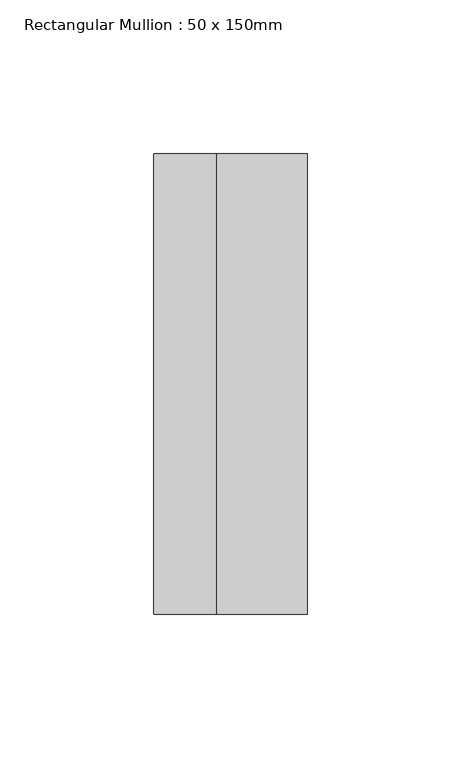
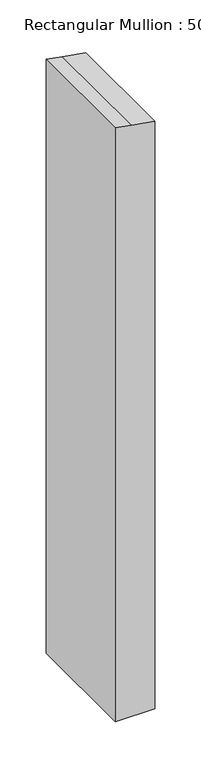
"""IFC4 building model written with IfcOpenShell, lengths in millimetres: member geometry, Rectangular Mullion : 50 x 150mm."""

import ifcopenshell
import ifcopenshell.guid

model = None  # the IFC model being written
_history = None  # IfcOwnerHistory: only IFC2X3 demands one
_inside = {}  # id of a spatial element -> (the spatial element, [elements in it])
_under = {}  # id of a project, library or spatial element -> (it, [spatial elements below it])
_declared = {}  # id of a project -> (the project, [libraries it declares])
_typed = {}  # id of a type object -> (the type object, [elements of that type])
_made_of = {}  # id of a material, layer set ... -> (it, [elements and type objects made of it])


def new_model(schema):
    """Start an empty IFC model of exactly this schema.

    Asked for "IFC4X3", IfcOpenShell would pick the latest addendum, in which some entities
    have other attributes; the version numbers below select the first issue.
    IFC2X3 requires an IfcOwnerHistory on every rooted entity: one is made here for all.
    """
    global model, _history
    if schema == "IFC4X3":
        model = ifcopenshell.file(schema_version=(4, 3, 0, 0))
    else:
        model = ifcopenshell.file(schema=schema)
    _inside.clear()
    _under.clear()
    _declared.clear()
    _typed.clear()
    _made_of.clear()
    _history = None
    if model.schema == "IFC2X3":
        org = make("IfcOrganization", Name="unknown")
        user = make(
            "IfcPersonAndOrganization",
            ThePerson=make("IfcPerson", FamilyName="unknown"),
            TheOrganization=org,
        )
        app = make(
            "IfcApplication",
            ApplicationDeveloper=org,
            Version="unknown",
            ApplicationFullName="unknown",
            ApplicationIdentifier="unknown",
        )
        _history = make(
            "IfcOwnerHistory",
            OwningUser=user,
            OwningApplication=app,
            ChangeAction="ADDED",
            CreationDate=0,
        )
    return model


def make(cls, **values):
    """One entity of the class cls with the attributes given. An attribute that is None is left unset."""
    return model.create_entity(
        cls, **{name: value for name, value in values.items() if value is not None}
    )


def rooted(cls, **values):
    """An entity with a GlobalId (a new one), such as an element, a storey or a relation."""
    return make(cls, GlobalId=ifcopenshell.guid.new(), OwnerHistory=_history, **values)


def si_unit(unit_type, name, prefix=None):
    """IfcSIUnit, for example si_unit("LENGTHUNIT", "METRE", prefix="MILLI")."""
    return make("IfcSIUnit", UnitType=unit_type, Prefix=prefix, Name=name)


def assignment(units):
    """IfcUnitAssignment: the units of a project."""
    return None if units is None else make("IfcUnitAssignment", Units=units)


def point(xyz):
    """IfcCartesianPoint."""
    return None if xyz is None else make("IfcCartesianPoint", Coordinates=xyz)


def direction(xyz):
    """IfcDirection."""
    return None if xyz is None else make("IfcDirection", DirectionRatios=xyz)


def frame(location, z_axis=None, x_axis=None):
    """IfcAxis2Placement3D, a coordinate frame: its origin and axes. An axis left out is left unset."""
    return make(
        "IfcAxis2Placement3D",
        Location=point(location),
        Axis=direction(z_axis),
        RefDirection=direction(x_axis),
    )


def origin():
    """The frame at (0, 0, 0) with its axes left unset."""
    return frame((0.0, 0.0, 0.0))


def place(relative_to, where):
    """IfcLocalPlacement: puts the frame where relative to a parent placement (None: the world)."""
    return make(
        "IfcLocalPlacement", PlacementRelTo=relative_to, RelativePlacement=where
    )


def context(
    kind, dimensions, precision=None, world=None, true_north=None, identifier=None
):
    """IfcGeometricRepresentationContext, for example the 3D "Model" context."""
    return make(
        "IfcGeometricRepresentationContext",
        ContextIdentifier=identifier,
        ContextType=kind,
        CoordinateSpaceDimension=dimensions,
        Precision=precision,
        WorldCoordinateSystem=world,
        TrueNorth=true_north,
    )


def project(units=None, contexts=None):
    """IfcProject with its units and contexts."""
    return rooted(
        "IfcProject",
        Name="project",
        RepresentationContexts=contexts,
        UnitsInContext=assignment(units),
    )


def spatial(cls, under=None, at=None, **own):
    """A site, building, storey or space (cls), placed at a placement, below another one or the project."""
    s = rooted(cls, ObjectPlacement=at, **own)
    if under is not None:
        _under.setdefault(under.id(), (under, []))[1].append(s)
    return s


def polyline(points):
    """IfcPolyline through the points."""
    return make("IfcPolyline", Points=[point(p) for p in points])


def outline(outer, holes=None, kind="AREA"):
    """IfcArbitraryClosedProfileDef: a profile drawn as a closed curve; with holes, ...WithVoids."""
    if holes is None:
        return make("IfcArbitraryClosedProfileDef", ProfileType=kind, OuterCurve=outer)
    return make(
        "IfcArbitraryProfileDefWithVoids",
        ProfileType=kind,
        OuterCurve=outer,
        InnerCurves=holes,
    )


def extrude(swept, where, along, depth):
    """IfcExtrudedAreaSolid: the profile swept, set in the frame where, extruded along a direction by depth."""
    return make(
        "IfcExtrudedAreaSolid",
        SweptArea=swept,
        Position=where,
        ExtrudedDirection=direction(along),
        Depth=depth,
    )


def shape(context_of_items, identifier, shape_type, items):
    """IfcShapeRepresentation: the items that make up one representation, for example the "Body"."""
    return make(
        "IfcShapeRepresentation",
        ContextOfItems=context_of_items,
        RepresentationIdentifier=identifier,
        RepresentationType=shape_type,
        Items=items,
    )


def source(mapping_origin, context_of_items, identifier, shape_type, items):
    """IfcRepresentationMap: a shape defined once, which mapped items show again and again."""
    return make(
        "IfcRepresentationMap",
        MappingOrigin=mapping_origin,
        MappedRepresentation=shape(context_of_items, identifier, shape_type, items),
    )


def transform(
    local_origin,
    x_axis=None,
    y_axis=None,
    z_axis=None,
    scale=None,
    scale2=None,
    scale3=None,
    uniform=True,
):
    """IfcCartesianTransformationOperator3D, or its non-uniform kind. x_axis, y_axis, z_axis: its Axis1, 2, 3."""
    if uniform:
        return make(
            "IfcCartesianTransformationOperator3D",
            Axis1=direction(x_axis),
            Axis2=direction(y_axis),
            LocalOrigin=point(local_origin),
            Scale=scale,
            Axis3=direction(z_axis),
        )
    return make(
        "IfcCartesianTransformationOperator3DnonUniform",
        Axis1=direction(x_axis),
        Axis2=direction(y_axis),
        LocalOrigin=point(local_origin),
        Scale=scale,
        Axis3=direction(z_axis),
        Scale2=scale2,
        Scale3=scale3,
    )


def mapped(mapping_source, mapping_target):
    """IfcMappedItem: shows the shape of a source again, moved by a transform."""
    return make(
        "IfcMappedItem", MappingSource=mapping_source, MappingTarget=mapping_target
    )


def made_of(thing, what):
    """Note that an element or type object is made of a material, layer set ...; save() writes the relation."""
    if what is not None:
        _made_of.setdefault(what.id(), (what, []))[1].append(thing)
    return thing


def element(
    cls,
    number,
    at=None,
    inside=None,
    cuts=None,
    type_object=None,
    material=None,
    context=None,
    identifier="Body",
    shape_type=None,
    held_by="IfcProductDefinitionShape",
    body=None,
    shapes=None,
    **own,
):
    """One element of the class cls, such as IfcWall. Its Tag is "e" and its number.

    at: its placement. inside: the storey or other place that contains it. cuts: it is an
    opening in that element (IfcRelVoidsElement). A single representation is given by context,
    identifier, shape_type and body (its items); several are given by shapes. held_by: the class
    of the entity that holds the representations. save() writes the other relations.
    """
    e = rooted(cls, Tag="e%d" % number, ObjectPlacement=at, **own)
    if body is not None:
        shapes = [shape(context, identifier, shape_type, body)]
    if shapes is not None:
        e.Representation = make(held_by, Representations=shapes)
    if inside is not None:
        _inside.setdefault(inside.id(), (inside, []))[1].append(e)
    if cuts is not None:
        rooted(
            "IfcRelVoidsElement", RelatingBuildingElement=cuts, RelatedOpeningElement=e
        )
    if type_object is not None:
        _typed.setdefault(type_object.id(), (type_object, []))[1].append(e)
    return made_of(e, material)


def aggregate(whole, parts):
    """IfcRelAggregates: a whole, such as a stair, and the parts it consists of."""
    return rooted("IfcRelAggregates", RelatingObject=whole, RelatedObjects=parts)


def save(model, path):
    """Write the relations noted so far, then the file.

    IfcRelAggregates (storeys below a building ...), IfcRelContainedInSpatialStructure (elements
    in a storey), IfcRelDefinesByType, IfcRelAssociatesMaterial and IfcRelDeclares: one each for
    every whole, place, type object, material and project.
    """
    for whole, parts in _under.values():
        aggregate(whole, parts)
    for where, things in _inside.values():
        rooted(
            "IfcRelContainedInSpatialStructure",
            RelatedElements=things,
            RelatingStructure=where,
        )
    for kind, things in _typed.values():
        rooted("IfcRelDefinesByType", RelatedObjects=things, RelatingType=kind)
    for what, things in _made_of.values():
        rooted("IfcRelAssociatesMaterial", RelatedObjects=things, RelatingMaterial=what)
    for by, libraries in _declared.values():
        rooted("IfcRelDeclares", RelatingContext=by, RelatedDefinitions=libraries)
    model.write(path)


def rectangular_mullion_50_x_150mm_6a3808df(model_context):
    return source(origin(), model_context, "Body", "SweptSolid", [
        extrude(outline(polyline([(-4.7938398, 25.0), (0.3798062, -4.3412044), (4.0225092, -25.0), (-783.9384156, -25.0), (-783.9384156, 25.0), (-4.7938398, 25.0)])), frame((0.0, -75.0, 0.0), z_axis=(0.0, 1.0, 0.0), x_axis=(0.0, 0.0, 1.0)), (0.0, 0.0, 1.0), 150.0),
    ])


if __name__ == "__main__":
    model = new_model("IFC4")
    model_context = context("Model", 3, world=origin())
    ifc_project = project(units=[si_unit("LENGTHUNIT", "METRE", prefix="MILLI")], contexts=[model_context])
    site = spatial("IfcSite", under=ifc_project)
    building = spatial("IfcBuilding", under=site)
    placement = place(None, origin())
    rectangular_mullion_50_x_150mm_shape = rectangular_mullion_50_x_150mm_6a3808df(model_context)
    element("IfcMember", 1, ObjectType="Rectangular Mullion : 50 x 150mm", at=placement, inside=building, context=model_context, shape_type="MappedRepresentation", body=[
        mapped(rectangular_mullion_50_x_150mm_shape, transform((0.0, 0.0, 0.0), x_axis=(1.0, 0.0, 0.0), y_axis=(0.0, 1.0, 0.0), z_axis=(0.0, 0.0, 1.0))),
    ])
    save(model, "model.ifc")

# Revit data of these elements
# Type "Rectangular Mullion : 50 x 150mm"
#   built-in parameter 1007304 = 0.492126 (stored number, unit not read)
#   built-in parameter 1007301 = 0.082021 (stored number, unit not read)
#   built-in parameter 1007300 = 0.082021 (stored number, unit not read)
# Element 1 (IfcMember, "Rectangular Mullion : 50 x 150mm")
#   Materials on its faces: "Aluminium"
# Materials
#   "Aluminium": class "Metal", colour RGB 247 247 247, transparency 0, Description = "Aluminium 6061", Cost = 0
